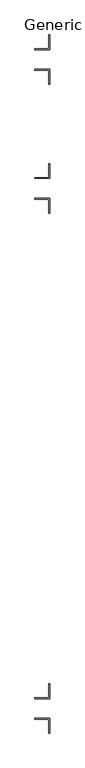
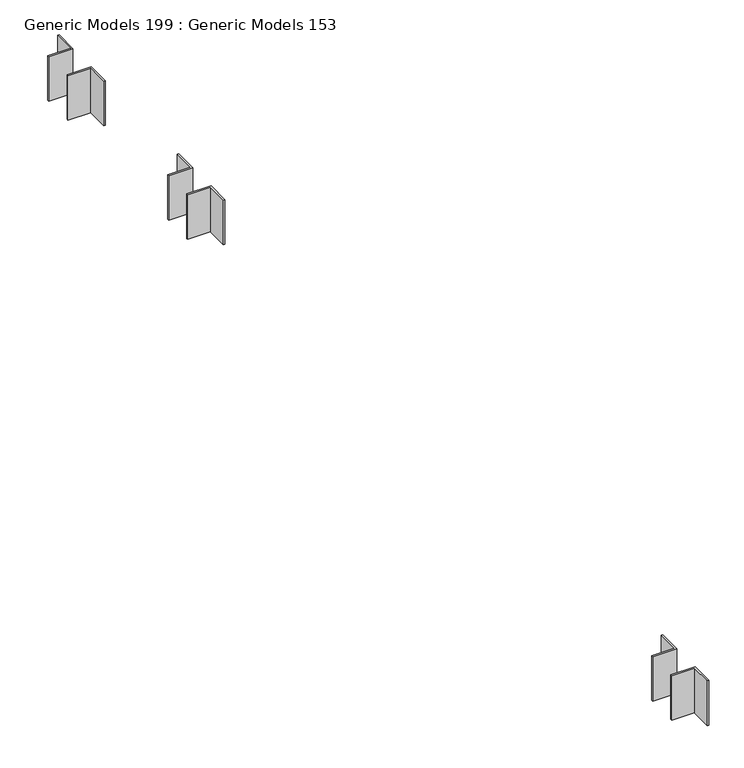
"""IFC4 building model written with IfcOpenShell, lengths in millimetres: proxy geometry, Generic Models 199 : Generic Models 153."""

import ifcopenshell
import ifcopenshell.guid

model = None  # the IFC model being written
_history = None  # IfcOwnerHistory: only IFC2X3 demands one
_inside = {}  # id of a spatial element -> (the spatial element, [elements in it])
_under = {}  # id of a project, library or spatial element -> (it, [spatial elements below it])
_declared = {}  # id of a project -> (the project, [libraries it declares])
_typed = {}  # id of a type object -> (the type object, [elements of that type])
_made_of = {}  # id of a material, layer set ... -> (it, [elements and type objects made of it])


def new_model(schema):
    """Start an empty IFC model of exactly this schema.

    Asked for "IFC4X3", IfcOpenShell would pick the latest addendum, in which some entities
    have other attributes; the version numbers below select the first issue.
    IFC2X3 requires an IfcOwnerHistory on every rooted entity: one is made here for all.
    """
    global model, _history
    if schema == "IFC4X3":
        model = ifcopenshell.file(schema_version=(4, 3, 0, 0))
    else:
        model = ifcopenshell.file(schema=schema)
    _inside.clear()
    _under.clear()
    _declared.clear()
    _typed.clear()
    _made_of.clear()
    _history = None
    if model.schema == "IFC2X3":
        org = make("IfcOrganization", Name="unknown")
        user = make(
            "IfcPersonAndOrganization",
            ThePerson=make("IfcPerson", FamilyName="unknown"),
            TheOrganization=org,
        )
        app = make(
            "IfcApplication",
            ApplicationDeveloper=org,
            Version="unknown",
            ApplicationFullName="unknown",
            ApplicationIdentifier="unknown",
        )
        _history = make(
            "IfcOwnerHistory",
            OwningUser=user,
            OwningApplication=app,
            ChangeAction="ADDED",
            CreationDate=0,
        )
    return model


def make(cls, **values):
    """One entity of the class cls with the attributes given. An attribute that is None is left unset."""
    return model.create_entity(
        cls, **{name: value for name, value in values.items() if value is not None}
    )


def rooted(cls, **values):
    """An entity with a GlobalId (a new one), such as an element, a storey or a relation."""
    return make(cls, GlobalId=ifcopenshell.guid.new(), OwnerHistory=_history, **values)


def si_unit(unit_type, name, prefix=None):
    """IfcSIUnit, for example si_unit("LENGTHUNIT", "METRE", prefix="MILLI")."""
    return make("IfcSIUnit", UnitType=unit_type, Prefix=prefix, Name=name)


def assignment(units):
    """IfcUnitAssignment: the units of a project."""
    return None if units is None else make("IfcUnitAssignment", Units=units)


def point(xyz):
    """IfcCartesianPoint."""
    return None if xyz is None else make("IfcCartesianPoint", Coordinates=xyz)


def direction(xyz):
    """IfcDirection."""
    return None if xyz is None else make("IfcDirection", DirectionRatios=xyz)


def frame(location, z_axis=None, x_axis=None):
    """IfcAxis2Placement3D, a coordinate frame: its origin and axes. An axis left out is left unset."""
    return make(
        "IfcAxis2Placement3D",
        Location=point(location),
        Axis=direction(z_axis),
        RefDirection=direction(x_axis),
    )


def origin():
    """The frame at (0, 0, 0) with its axes left unset."""
    return frame((0.0, 0.0, 0.0))


def place(relative_to, where):
    """IfcLocalPlacement: puts the frame where relative to a parent placement (None: the world)."""
    return make(
        "IfcLocalPlacement", PlacementRelTo=relative_to, RelativePlacement=where
    )


def context(
    kind, dimensions, precision=None, world=None, true_north=None, identifier=None
):
    """IfcGeometricRepresentationContext, for example the 3D "Model" context."""
    return make(
        "IfcGeometricRepresentationContext",
        ContextIdentifier=identifier,
        ContextType=kind,
        CoordinateSpaceDimension=dimensions,
        Precision=precision,
        WorldCoordinateSystem=world,
        TrueNorth=true_north,
    )


def project(units=None, contexts=None):
    """IfcProject with its units and contexts."""
    return rooted(
        "IfcProject",
        Name="project",
        RepresentationContexts=contexts,
        UnitsInContext=assignment(units),
    )


def spatial(cls, under=None, at=None, **own):
    """A site, building, storey or space (cls), placed at a placement, below another one or the project."""
    s = rooted(cls, ObjectPlacement=at, **own)
    if under is not None:
        _under.setdefault(under.id(), (under, []))[1].append(s)
    return s


def polyline(points):
    """IfcPolyline through the points."""
    return make("IfcPolyline", Points=[point(p) for p in points])


def outline(outer, holes=None, kind="AREA"):
    """IfcArbitraryClosedProfileDef: a profile drawn as a closed curve; with holes, ...WithVoids."""
    if holes is None:
        return make("IfcArbitraryClosedProfileDef", ProfileType=kind, OuterCurve=outer)
    return make(
        "IfcArbitraryProfileDefWithVoids",
        ProfileType=kind,
        OuterCurve=outer,
        InnerCurves=holes,
    )


def extrude(swept, where, along, depth):
    """IfcExtrudedAreaSolid: the profile swept, set in the frame where, extruded along a direction by depth."""
    return make(
        "IfcExtrudedAreaSolid",
        SweptArea=swept,
        Position=where,
        ExtrudedDirection=direction(along),
        Depth=depth,
    )


def shape(context_of_items, identifier, shape_type, items):
    """IfcShapeRepresentation: the items that make up one representation, for example the "Body"."""
    return make(
        "IfcShapeRepresentation",
        ContextOfItems=context_of_items,
        RepresentationIdentifier=identifier,
        RepresentationType=shape_type,
        Items=items,
    )


def source(mapping_origin, context_of_items, identifier, shape_type, items):
    """IfcRepresentationMap: a shape defined once, which mapped items show again and again."""
    return make(
        "IfcRepresentationMap",
        MappingOrigin=mapping_origin,
        MappedRepresentation=shape(context_of_items, identifier, shape_type, items),
    )


def transform(
    local_origin,
    x_axis=None,
    y_axis=None,
    z_axis=None,
    scale=None,
    scale2=None,
    scale3=None,
    uniform=True,
):
    """IfcCartesianTransformationOperator3D, or its non-uniform kind. x_axis, y_axis, z_axis: its Axis1, 2, 3."""
    if uniform:
        return make(
            "IfcCartesianTransformationOperator3D",
            Axis1=direction(x_axis),
            Axis2=direction(y_axis),
            LocalOrigin=point(local_origin),
            Scale=scale,
            Axis3=direction(z_axis),
        )
    return make(
        "IfcCartesianTransformationOperator3DnonUniform",
        Axis1=direction(x_axis),
        Axis2=direction(y_axis),
        LocalOrigin=point(local_origin),
        Scale=scale,
        Axis3=direction(z_axis),
        Scale2=scale2,
        Scale3=scale3,
    )


def mapped(mapping_source, mapping_target):
    """IfcMappedItem: shows the shape of a source again, moved by a transform."""
    return make(
        "IfcMappedItem", MappingSource=mapping_source, MappingTarget=mapping_target
    )


def made_of(thing, what):
    """Note that an element or type object is made of a material, layer set ...; save() writes the relation."""
    if what is not None:
        _made_of.setdefault(what.id(), (what, []))[1].append(thing)
    return thing


def element(
    cls,
    number,
    at=None,
    inside=None,
    cuts=None,
    type_object=None,
    material=None,
    context=None,
    identifier="Body",
    shape_type=None,
    held_by="IfcProductDefinitionShape",
    body=None,
    shapes=None,
    **own,
):
    """One element of the class cls, such as IfcWall. Its Tag is "e" and its number.

    at: its placement. inside: the storey or other place that contains it. cuts: it is an
    opening in that element (IfcRelVoidsElement). A single representation is given by context,
    identifier, shape_type and body (its items); several are given by shapes. held_by: the class
    of the entity that holds the representations. save() writes the other relations.
    """
    e = rooted(cls, Tag="e%d" % number, ObjectPlacement=at, **own)
    if body is not None:
        shapes = [shape(context, identifier, shape_type, body)]
    if shapes is not None:
        e.Representation = make(held_by, Representations=shapes)
    if inside is not None:
        _inside.setdefault(inside.id(), (inside, []))[1].append(e)
    if cuts is not None:
        rooted(
            "IfcRelVoidsElement", RelatingBuildingElement=cuts, RelatedOpeningElement=e
        )
    if type_object is not None:
        _typed.setdefault(type_object.id(), (type_object, []))[1].append(e)
    return made_of(e, material)


def aggregate(whole, parts):
    """IfcRelAggregates: a whole, such as a stair, and the parts it consists of."""
    return rooted("IfcRelAggregates", RelatingObject=whole, RelatedObjects=parts)


def save(model, path):
    """Write the relations noted so far, then the file.

    IfcRelAggregates (storeys below a building ...), IfcRelContainedInSpatialStructure (elements
    in a storey), IfcRelDefinesByType, IfcRelAssociatesMaterial and IfcRelDeclares: one each for
    every whole, place, type object, material and project.
    """
    for whole, parts in _under.values():
        aggregate(whole, parts)
    for where, things in _inside.values():
        rooted(
            "IfcRelContainedInSpatialStructure",
            RelatedElements=things,
            RelatingStructure=where,
        )
    for kind, things in _typed.values():
        rooted("IfcRelDefinesByType", RelatedObjects=things, RelatingType=kind)
    for what, things in _made_of.values():
        rooted("IfcRelAssociatesMaterial", RelatedObjects=things, RelatingMaterial=what)
    for by, libraries in _declared.values():
        rooted("IfcRelDeclares", RelatingContext=by, RelatedDefinitions=libraries)
    model.write(path)


def generic_models_199_generic_models_153_dd3a872e(model_context):
    return source(origin(), model_context, "Body", "SweptSolid", [
        extrude(outline(polyline([(31813.4846032, 30988.6531612), (31821.4221032, 30988.6531612), (31821.4221032, 30860.0656612), (31691.2471032, 30860.0656612), (31691.2471032, 30868.0031612), (31813.4846032, 30868.0031612), (31813.4846032, 30988.6531612)])), frame((0.0, 0.0, 268836.775), z_axis=(0.0, 0.0, 1.0), x_axis=(1.0, 0.0, 0.0)), (0.0, 0.0, 1.0), 254.0),
        extrude(outline(polyline([(31813.4846032, 30560.0281612), (31813.4846032, 30680.6781612), (31691.2471032, 30680.6781612), (31691.2471032, 30688.6156612), (31821.4221032, 30688.6156612), (31821.4221032, 30560.0281612), (31813.4846032, 30560.0281612)])), frame((0.0, 0.0, 268836.775), z_axis=(0.0, 0.0, 1.0), x_axis=(1.0, 0.0, 0.0)), (0.0, 0.0, 1.0), 254.0),
        extrude(outline(polyline([(31813.4846032, 35504.1332942), (31821.4221032, 35504.1332942), (31821.4221032, 35375.5457942), (31691.2471032, 35375.5457942), (31691.2471032, 35383.4832942), (31813.4846032, 35383.4832942), (31813.4846032, 35504.1332942)])), frame((0.0, 0.0, 268836.775), z_axis=(0.0, 0.0, 1.0), x_axis=(1.0, 0.0, 0.0)), (0.0, 0.0, 1.0), 254.0),
        extrude(outline(polyline([(31813.4846032, 35075.5082942), (31813.4846032, 35196.1582942), (31691.2471032, 35196.1582942), (31691.2471032, 35204.0957942), (31821.4221032, 35204.0957942), (31821.4221032, 35075.5082942), (31813.4846032, 35075.5082942)])), frame((0.0, 0.0, 268836.775), z_axis=(0.0, 0.0, 1.0), x_axis=(1.0, 0.0, 0.0)), (0.0, 0.0, 1.0), 254.0),
        extrude(outline(polyline([(31813.4846032, 36621.7332942), (31821.4221032, 36621.7332942), (31821.4221032, 36493.1457942), (31691.2471032, 36493.1457942), (31691.2471032, 36501.0832942), (31813.4846032, 36501.0832942), (31813.4846032, 36621.7332942)])), frame((0.0, 0.0, 268836.775), z_axis=(0.0, 0.0, 1.0), x_axis=(1.0, 0.0, 0.0)), (0.0, 0.0, 1.0), 254.0),
        extrude(outline(polyline([(31813.4846032, 36193.1082942), (31813.4846032, 36313.7582942), (31691.2471032, 36313.7582942), (31691.2471032, 36321.6957942), (31821.4221032, 36321.6957942), (31821.4221032, 36193.1082942), (31813.4846032, 36193.1082942)])), frame((0.0, 0.0, 268836.775), z_axis=(0.0, 0.0, 1.0), x_axis=(1.0, 0.0, 0.0)), (0.0, 0.0, 1.0), 254.0),
    ])


if __name__ == "__main__":
    model = new_model("IFC4")
    model_context = context("Model", 3, world=origin())
    ifc_project = project(units=[si_unit("LENGTHUNIT", "METRE", prefix="MILLI")], contexts=[model_context])
    site = spatial("IfcSite", under=ifc_project)
    building = spatial("IfcBuilding", under=site)
    placement = place(None, origin())
    generic_models_199_generic_models_153_shape = generic_models_199_generic_models_153_dd3a872e(model_context)
    element("IfcBuildingElementProxy", 1, Name="Generic Models 199 : Generic Models 153", ObjectType="Generic Models 199 : Generic Models 153", at=placement, inside=building, context=model_context, shape_type="MappedRepresentation", body=[
        mapped(generic_models_199_generic_models_153_shape, transform((0.0, 0.0, 0.0), x_axis=(1.0, 0.0, 0.0), y_axis=(0.0, 1.0, 0.0), z_axis=(0.0, 0.0, 1.0))),
    ])
    save(model, "model.ifc")
